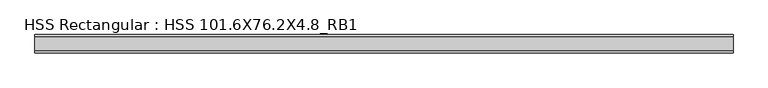
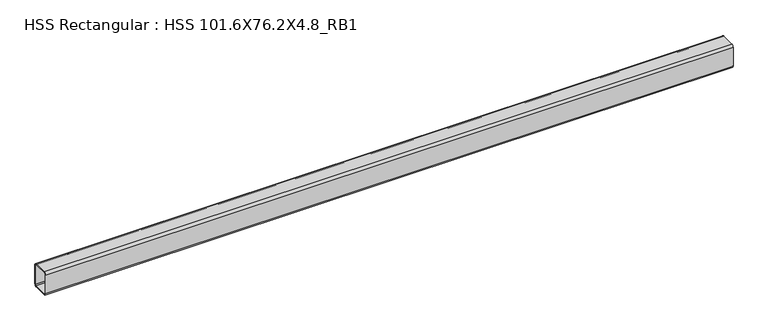
"""IFC4 building model written with IfcOpenShell, lengths in millimetres: beam geometry, HSS Rectangular : HSS 101.6X76.2X4.8_RB1."""

import ifcopenshell
import ifcopenshell.guid

model = None  # the IFC model being written
_history = None  # IfcOwnerHistory: only IFC2X3 demands one
_inside = {}  # id of a spatial element -> (the spatial element, [elements in it])
_under = {}  # id of a project, library or spatial element -> (it, [spatial elements below it])
_declared = {}  # id of a project -> (the project, [libraries it declares])
_typed = {}  # id of a type object -> (the type object, [elements of that type])
_made_of = {}  # id of a material, layer set ... -> (it, [elements and type objects made of it])


def new_model(schema):
    """Start an empty IFC model of exactly this schema.

    Asked for "IFC4X3", IfcOpenShell would pick the latest addendum, in which some entities
    have other attributes; the version numbers below select the first issue.
    IFC2X3 requires an IfcOwnerHistory on every rooted entity: one is made here for all.
    """
    global model, _history
    if schema == "IFC4X3":
        model = ifcopenshell.file(schema_version=(4, 3, 0, 0))
    else:
        model = ifcopenshell.file(schema=schema)
    _inside.clear()
    _under.clear()
    _declared.clear()
    _typed.clear()
    _made_of.clear()
    _history = None
    if model.schema == "IFC2X3":
        org = make("IfcOrganization", Name="unknown")
        user = make(
            "IfcPersonAndOrganization",
            ThePerson=make("IfcPerson", FamilyName="unknown"),
            TheOrganization=org,
        )
        app = make(
            "IfcApplication",
            ApplicationDeveloper=org,
            Version="unknown",
            ApplicationFullName="unknown",
            ApplicationIdentifier="unknown",
        )
        _history = make(
            "IfcOwnerHistory",
            OwningUser=user,
            OwningApplication=app,
            ChangeAction="ADDED",
            CreationDate=0,
        )
    return model


def make(cls, **values):
    """One entity of the class cls with the attributes given. An attribute that is None is left unset."""
    return model.create_entity(
        cls, **{name: value for name, value in values.items() if value is not None}
    )


def rooted(cls, **values):
    """An entity with a GlobalId (a new one), such as an element, a storey or a relation."""
    return make(cls, GlobalId=ifcopenshell.guid.new(), OwnerHistory=_history, **values)


def si_unit(unit_type, name, prefix=None):
    """IfcSIUnit, for example si_unit("LENGTHUNIT", "METRE", prefix="MILLI")."""
    return make("IfcSIUnit", UnitType=unit_type, Prefix=prefix, Name=name)


def assignment(units):
    """IfcUnitAssignment: the units of a project."""
    return None if units is None else make("IfcUnitAssignment", Units=units)


def point(xyz):
    """IfcCartesianPoint."""
    return None if xyz is None else make("IfcCartesianPoint", Coordinates=xyz)


def direction(xyz):
    """IfcDirection."""
    return None if xyz is None else make("IfcDirection", DirectionRatios=xyz)


def frame(location, z_axis=None, x_axis=None):
    """IfcAxis2Placement3D, a coordinate frame: its origin and axes. An axis left out is left unset."""
    return make(
        "IfcAxis2Placement3D",
        Location=point(location),
        Axis=direction(z_axis),
        RefDirection=direction(x_axis),
    )


def frame_2d(location, x_axis=None):
    """IfcAxis2Placement2D, a coordinate frame in the plane: its origin and x axis."""
    return make(
        "IfcAxis2Placement2D", Location=point(location), RefDirection=direction(x_axis)
    )


def origin():
    """The frame at (0, 0, 0) with its axes left unset."""
    return frame((0.0, 0.0, 0.0))


def place(relative_to, where):
    """IfcLocalPlacement: puts the frame where relative to a parent placement (None: the world)."""
    return make(
        "IfcLocalPlacement", PlacementRelTo=relative_to, RelativePlacement=where
    )


def context(
    kind, dimensions, precision=None, world=None, true_north=None, identifier=None
):
    """IfcGeometricRepresentationContext, for example the 3D "Model" context."""
    return make(
        "IfcGeometricRepresentationContext",
        ContextIdentifier=identifier,
        ContextType=kind,
        CoordinateSpaceDimension=dimensions,
        Precision=precision,
        WorldCoordinateSystem=world,
        TrueNorth=true_north,
    )


def project(units=None, contexts=None):
    """IfcProject with its units and contexts."""
    return rooted(
        "IfcProject",
        Name="project",
        RepresentationContexts=contexts,
        UnitsInContext=assignment(units),
    )


def spatial(cls, under=None, at=None, **own):
    """A site, building, storey or space (cls), placed at a placement, below another one or the project."""
    s = rooted(cls, ObjectPlacement=at, **own)
    if under is not None:
        _under.setdefault(under.id(), (under, []))[1].append(s)
    return s


def polyline(points):
    """IfcPolyline through the points."""
    return make("IfcPolyline", Points=[point(p) for p in points])


def circle_curve(where, radius):
    """IfcCircle in the frame where."""
    return make("IfcCircle", Position=where, Radius=radius)


def trimmed(basis, trim1, trim2, sense, master):
    """IfcTrimmedCurve: the piece of a basis curve between two trims."""
    return make(
        "IfcTrimmedCurve",
        BasisCurve=basis,
        Trim1=trim1,
        Trim2=trim2,
        SenseAgreement=sense,
        MasterRepresentation=master,
    )


def segment(curve, same_sense, transition):
    """IfcCompositeCurveSegment."""
    return make(
        "IfcCompositeCurveSegment",
        Transition=transition,
        SameSense=same_sense,
        ParentCurve=curve,
    )


def composite_curve(segments, self_intersect=None):
    """IfcCompositeCurve: segments joined end to end."""
    return make("IfcCompositeCurve", Segments=segments, SelfIntersect=self_intersect)


def outline(outer, holes=None, kind="AREA"):
    """IfcArbitraryClosedProfileDef: a profile drawn as a closed curve; with holes, ...WithVoids."""
    if holes is None:
        return make("IfcArbitraryClosedProfileDef", ProfileType=kind, OuterCurve=outer)
    return make(
        "IfcArbitraryProfileDefWithVoids",
        ProfileType=kind,
        OuterCurve=outer,
        InnerCurves=holes,
    )


def extrude(swept, where, along, depth):
    """IfcExtrudedAreaSolid: the profile swept, set in the frame where, extruded along a direction by depth."""
    return make(
        "IfcExtrudedAreaSolid",
        SweptArea=swept,
        Position=where,
        ExtrudedDirection=direction(along),
        Depth=depth,
    )


def shape(context_of_items, identifier, shape_type, items):
    """IfcShapeRepresentation: the items that make up one representation, for example the "Body"."""
    return make(
        "IfcShapeRepresentation",
        ContextOfItems=context_of_items,
        RepresentationIdentifier=identifier,
        RepresentationType=shape_type,
        Items=items,
    )


def source(mapping_origin, context_of_items, identifier, shape_type, items):
    """IfcRepresentationMap: a shape defined once, which mapped items show again and again."""
    return make(
        "IfcRepresentationMap",
        MappingOrigin=mapping_origin,
        MappedRepresentation=shape(context_of_items, identifier, shape_type, items),
    )


def transform(
    local_origin,
    x_axis=None,
    y_axis=None,
    z_axis=None,
    scale=None,
    scale2=None,
    scale3=None,
    uniform=True,
):
    """IfcCartesianTransformationOperator3D, or its non-uniform kind. x_axis, y_axis, z_axis: its Axis1, 2, 3."""
    if uniform:
        return make(
            "IfcCartesianTransformationOperator3D",
            Axis1=direction(x_axis),
            Axis2=direction(y_axis),
            LocalOrigin=point(local_origin),
            Scale=scale,
            Axis3=direction(z_axis),
        )
    return make(
        "IfcCartesianTransformationOperator3DnonUniform",
        Axis1=direction(x_axis),
        Axis2=direction(y_axis),
        LocalOrigin=point(local_origin),
        Scale=scale,
        Axis3=direction(z_axis),
        Scale2=scale2,
        Scale3=scale3,
    )


def mapped(mapping_source, mapping_target):
    """IfcMappedItem: shows the shape of a source again, moved by a transform."""
    return make(
        "IfcMappedItem", MappingSource=mapping_source, MappingTarget=mapping_target
    )


def made_of(thing, what):
    """Note that an element or type object is made of a material, layer set ...; save() writes the relation."""
    if what is not None:
        _made_of.setdefault(what.id(), (what, []))[1].append(thing)
    return thing


def element(
    cls,
    number,
    at=None,
    inside=None,
    cuts=None,
    type_object=None,
    material=None,
    context=None,
    identifier="Body",
    shape_type=None,
    held_by="IfcProductDefinitionShape",
    body=None,
    shapes=None,
    **own,
):
    """One element of the class cls, such as IfcWall. Its Tag is "e" and its number.

    at: its placement. inside: the storey or other place that contains it. cuts: it is an
    opening in that element (IfcRelVoidsElement). A single representation is given by context,
    identifier, shape_type and body (its items); several are given by shapes. held_by: the class
    of the entity that holds the representations. save() writes the other relations.
    """
    e = rooted(cls, Tag="e%d" % number, ObjectPlacement=at, **own)
    if body is not None:
        shapes = [shape(context, identifier, shape_type, body)]
    if shapes is not None:
        e.Representation = make(held_by, Representations=shapes)
    if inside is not None:
        _inside.setdefault(inside.id(), (inside, []))[1].append(e)
    if cuts is not None:
        rooted(
            "IfcRelVoidsElement", RelatingBuildingElement=cuts, RelatedOpeningElement=e
        )
    if type_object is not None:
        _typed.setdefault(type_object.id(), (type_object, []))[1].append(e)
    return made_of(e, material)


def aggregate(whole, parts):
    """IfcRelAggregates: a whole, such as a stair, and the parts it consists of."""
    return rooted("IfcRelAggregates", RelatingObject=whole, RelatedObjects=parts)


def save(model, path):
    """Write the relations noted so far, then the file.

    IfcRelAggregates (storeys below a building ...), IfcRelContainedInSpatialStructure (elements
    in a storey), IfcRelDefinesByType, IfcRelAssociatesMaterial and IfcRelDeclares: one each for
    every whole, place, type object, material and project.
    """
    for whole, parts in _under.values():
        aggregate(whole, parts)
    for where, things in _inside.values():
        rooted(
            "IfcRelContainedInSpatialStructure",
            RelatedElements=things,
            RelatingStructure=where,
        )
    for kind, things in _typed.values():
        rooted("IfcRelDefinesByType", RelatedObjects=things, RelatingType=kind)
    for what, things in _made_of.values():
        rooted("IfcRelAssociatesMaterial", RelatedObjects=things, RelatingMaterial=what)
    for by, libraries in _declared.values():
        rooted("IfcRelDeclares", RelatingContext=by, RelatedDefinitions=libraries)
    model.write(path)


def hss_rectangular_hss_101_6x76_2x4_8_rb1_6d8b6784(model_context):
    return source(origin(), model_context, "Body", "SweptSolid", [
        extrude(outline(composite_curve([segment(trimmed(circle_curve(frame_2d((-28.575, 41.275)), 9.525), [point((-38.1, 41.275))], [point((-28.575, 50.8))], False, "CARTESIAN"), True, "CONTINUOUS"), segment(polyline([(-28.575, 50.8), (28.575, 50.8)]), True, "CONTINUOUS"), segment(trimmed(circle_curve(frame_2d((28.575, 41.275)), 9.525), [point((28.575, 50.8))], [point((38.1, 41.275))], False, "CARTESIAN"), True, "CONTINUOUS"), segment(polyline([(38.1, 41.275), (38.1, -41.275)]), True, "CONTINUOUS"), segment(trimmed(circle_curve(frame_2d((28.575, -41.275)), 9.525), [point((38.1, -41.275))], [point((28.575, -50.8))], False, "CARTESIAN"), True, "CONTINUOUS"), segment(polyline([(28.575, -50.8), (-28.575, -50.8)]), True, "CONTINUOUS"), segment(trimmed(circle_curve(frame_2d((-28.575, -41.275)), 9.525), [point((-28.575, -50.8))], [point((-38.1, -41.275))], False, "CARTESIAN"), True, "CONTINUOUS"), segment(polyline([(-38.1, -41.275), (-38.1, 41.275)]), True, "CONTINUOUS")], self_intersect=False), holes=[composite_curve([segment(polyline([(28.575, 46.0375), (-28.575, 46.0375)]), True, "CONTINUOUS"), segment(trimmed(circle_curve(frame_2d((-28.575, 41.275)), 4.7625), [point((-28.575, 46.0375))], [point((-33.3375, 41.275))], True, "CARTESIAN"), True, "CONTINUOUS"), segment(polyline([(-33.3375, 41.275), (-33.3375, -41.275)]), True, "CONTINUOUS"), segment(trimmed(circle_curve(frame_2d((-28.575, -41.275)), 4.7625), [point((-33.3375, -41.275))], [point((-28.575, -46.0375))], True, "CARTESIAN"), True, "CONTINUOUS"), segment(polyline([(-28.575, -46.0375), (28.575, -46.0375)]), True, "CONTINUOUS"), segment(trimmed(circle_curve(frame_2d((28.575, -41.275)), 4.7625), [point((28.575, -46.0375))], [point((33.3375, -41.275))], True, "CARTESIAN"), True, "CONTINUOUS"), segment(polyline([(33.3375, -41.275), (33.3375, 41.275)]), True, "CONTINUOUS"), segment(trimmed(circle_curve(frame_2d((28.575, 41.275)), 4.7625), [point((33.3375, 41.275))], [point((28.575, 46.0375))], True, "CARTESIAN"), True, "CONTINUOUS")], self_intersect=False)]), frame((-1474.1250006, 0.0, 0.0), z_axis=(1.0, 0.0, 0.0), x_axis=(0.0, 1.0, 0.0)), (0.0, 0.0, 1.0), 2884.7500012),
    ])


if __name__ == "__main__":
    model = new_model("IFC4")
    model_context = context("Model", 3, world=origin())
    ifc_project = project(units=[si_unit("LENGTHUNIT", "METRE", prefix="MILLI")], contexts=[model_context])
    site = spatial("IfcSite", under=ifc_project)
    building = spatial("IfcBuilding", under=site)
    placement = place(None, origin())
    hss_rectangular_hss_101_6x76_2x4_8_rb1_shape = hss_rectangular_hss_101_6x76_2x4_8_rb1_6d8b6784(model_context)
    element("IfcBeam", 1, ObjectType="HSS Rectangular : HSS 101.6X76.2X4.8_RB1", at=placement, inside=building, context=model_context, shape_type="MappedRepresentation", body=[
        mapped(hss_rectangular_hss_101_6x76_2x4_8_rb1_shape, transform((0.0, 0.0, 0.0), x_axis=(1.0, 0.0, 0.0), y_axis=(0.0, 1.0, 0.0), z_axis=(0.0, 0.0, 1.0))),
    ])
    save(model, "model.ifc")

# Revit data of these elements
# Type "HSS Rectangular : HSS 101.6X76.2X4.8_RB1"
#   Section Name Key = "HSS 4X3X3/16"
#   Assembly Code = "B10"
#   Width = 7.62 cm
#   Wall Nominal Thickness = 0.4763 cm
#   Wall Design Thickness = 0.442 cm
#   Torsional Moment of Inertia = 260.561 cm⁴
#   Torsional Modulus = 61.2876 cm³
#   Section Area = 14.4516 cm²
#   Plastic Modulus weak axis = 40.3122 cm³
#   Plastic Modulus strong axis = 49.1612 cm³
#   Perimeter = 0.881482 m²/m
#   Outer Fillet = 0.9525 cm
#   Nominal Weight = 12.1285 kgf/m
#   Moment of Inertia weak axis = 131.529 cm⁴
#   Moment of Inertia strong axis = 205.202 cm⁴
#   Inner Fillet = 0.4763 cm
#   Height = 10.16 cm
#   Elastic Modulus weak axis = 34.4128 cm³
#   Elastic Modulus strong axis = 40.476 cm³
#   Centroid Vertical = 5.08 cm
#   Centroid Horizontal = 3.81 cm
#   Length [instance default] = 1524 mm
#   Structural Material [instance default] = Steel ASTM A500, Grade B, Rectangular and Square
#   Principal Axes Angle = 0
# Element 1 (IfcBeam, "HSS Rectangular : HSS 101.6X76.2X4.8_RB1")
#   Structural Material = Steel ASTM A992
#   Materials on its faces: "Steel ASTM A992"
# Materials
#   "Steel ASTM A500, Grade B, Rectangular and Square": class "Metal", colour RGB 199 199 199, transparency 0, Description = "Carbon steel", Cost = 0
#   "Steel ASTM A992": class "Metal", colour RGB 199 199 199, transparency 0, Description = "Structural steel 50ksi", Cost = 0
